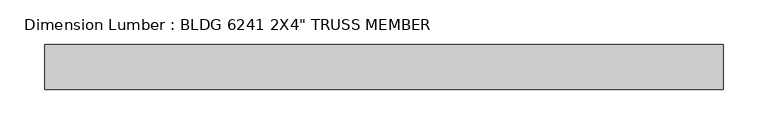
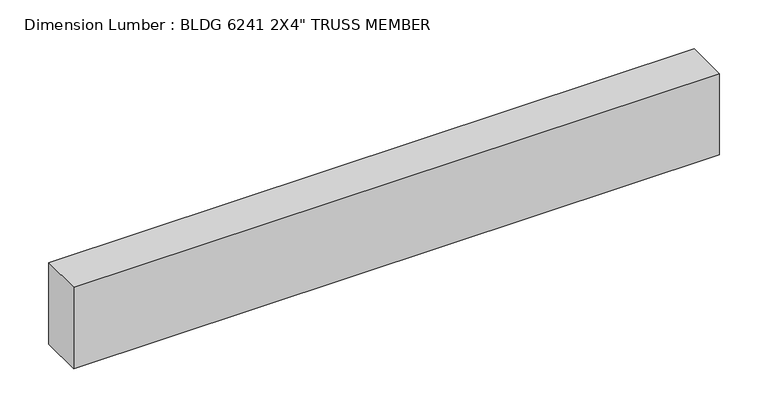
"""IFC4 building model written with IfcOpenShell, lengths in millimetres: beam geometry."""

from ifc_helpers import new_model, si_unit, frame, origin, place, context, project, spatial, polyline, outline, extrude, source, transform, mapped, element, save


def beam_54dd7b45(model_context):
    return source(origin(), model_context, "Body", "SweptSolid", [
        extrude(outline(polyline([(393.7, -25.4), (-368.3, -25.4), (-368.3, 25.4), (393.7, 25.4), (393.7, -25.4)])), frame((0.0, 0.0, -50.8), z_axis=(0.0, 0.0, 1.0), x_axis=(1.0, 0.0, 0.0)), (0.0, 0.0, 1.0), 101.6),
    ])


if __name__ == "__main__":
    model = new_model("IFC4")
    model_context = context("Model", 3, world=origin())
    ifc_project = project(units=[si_unit("LENGTHUNIT", "METRE", prefix="MILLI")], contexts=[model_context])
    site = spatial("IfcSite", under=ifc_project)
    building = spatial("IfcBuilding", under=site)
    placement = place(None, origin())
    beam_shape = beam_54dd7b45(model_context)
    element("IfcBeam", 1, ObjectType="Dimension Lumber : BLDG 6241 2X4\" TRUSS MEMBER", at=placement, inside=building, context=model_context, shape_type="MappedRepresentation", body=[
        mapped(beam_shape, transform((0.0, 0.0, 0.0), x_axis=(1.0, 0.0, 0.0), y_axis=(0.0, 1.0, 0.0), z_axis=(0.0, 0.0, 1.0))),
    ])
    save(model, "model.ifc")

# Revit data of these elements
# Type "Dimension Lumber : BLDG 6241 2X4\" TRUSS MEMBER"
#   Assembly Code = "B10"
#   A = 0.273472 SF
#   Length [instance default] = 5' - 0"
#   b = 0' - 2"
#   d = 0' - 4"
#   Structural Material [instance default] = Softwood, Lumber
# Element 1 (IfcBeam, "Dimension Lumber : BLDG 6241 2X4\" TRUSS MEMBER")
#   Materials on its faces: "Softwood, Lumber"
# Materials
#   "Softwood, Lumber": class "Wood", colour RGB 223 192 134, transparency 0, Description = "Pinus Echinata", Cost = 0
